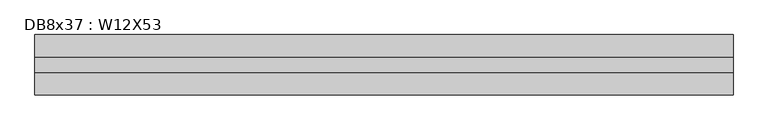
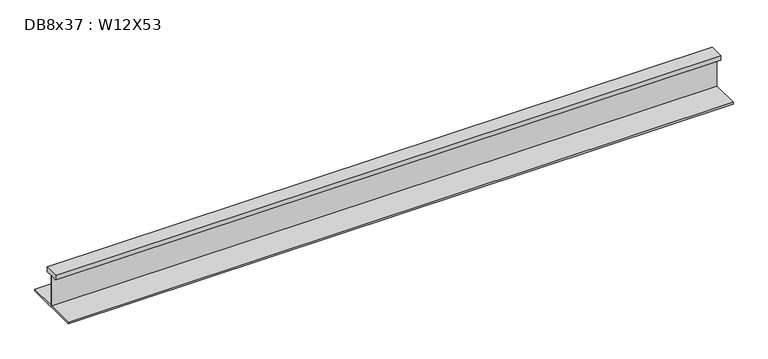
"""IFC4 building model written with IfcOpenShell, lengths in millimetres: beam geometry, DB8x37 : W12X53."""

import ifcopenshell
import ifcopenshell.guid

model = None  # the IFC model being written
_history = None  # IfcOwnerHistory: only IFC2X3 demands one
_inside = {}  # id of a spatial element -> (the spatial element, [elements in it])
_under = {}  # id of a project, library or spatial element -> (it, [spatial elements below it])
_declared = {}  # id of a project -> (the project, [libraries it declares])
_typed = {}  # id of a type object -> (the type object, [elements of that type])
_made_of = {}  # id of a material, layer set ... -> (it, [elements and type objects made of it])


def new_model(schema):
    """Start an empty IFC model of exactly this schema.

    Asked for "IFC4X3", IfcOpenShell would pick the latest addendum, in which some entities
    have other attributes; the version numbers below select the first issue.
    IFC2X3 requires an IfcOwnerHistory on every rooted entity: one is made here for all.
    """
    global model, _history
    if schema == "IFC4X3":
        model = ifcopenshell.file(schema_version=(4, 3, 0, 0))
    else:
        model = ifcopenshell.file(schema=schema)
    _inside.clear()
    _under.clear()
    _declared.clear()
    _typed.clear()
    _made_of.clear()
    _history = None
    if model.schema == "IFC2X3":
        org = make("IfcOrganization", Name="unknown")
        user = make(
            "IfcPersonAndOrganization",
            ThePerson=make("IfcPerson", FamilyName="unknown"),
            TheOrganization=org,
        )
        app = make(
            "IfcApplication",
            ApplicationDeveloper=org,
            Version="unknown",
            ApplicationFullName="unknown",
            ApplicationIdentifier="unknown",
        )
        _history = make(
            "IfcOwnerHistory",
            OwningUser=user,
            OwningApplication=app,
            ChangeAction="ADDED",
            CreationDate=0,
        )
    return model


def make(cls, **values):
    """One entity of the class cls with the attributes given. An attribute that is None is left unset."""
    return model.create_entity(
        cls, **{name: value for name, value in values.items() if value is not None}
    )


def rooted(cls, **values):
    """An entity with a GlobalId (a new one), such as an element, a storey or a relation."""
    return make(cls, GlobalId=ifcopenshell.guid.new(), OwnerHistory=_history, **values)


def si_unit(unit_type, name, prefix=None):
    """IfcSIUnit, for example si_unit("LENGTHUNIT", "METRE", prefix="MILLI")."""
    return make("IfcSIUnit", UnitType=unit_type, Prefix=prefix, Name=name)


def assignment(units):
    """IfcUnitAssignment: the units of a project."""
    return None if units is None else make("IfcUnitAssignment", Units=units)


def point(xyz):
    """IfcCartesianPoint."""
    return None if xyz is None else make("IfcCartesianPoint", Coordinates=xyz)


def direction(xyz):
    """IfcDirection."""
    return None if xyz is None else make("IfcDirection", DirectionRatios=xyz)


def frame(location, z_axis=None, x_axis=None):
    """IfcAxis2Placement3D, a coordinate frame: its origin and axes. An axis left out is left unset."""
    return make(
        "IfcAxis2Placement3D",
        Location=point(location),
        Axis=direction(z_axis),
        RefDirection=direction(x_axis),
    )


def origin():
    """The frame at (0, 0, 0) with its axes left unset."""
    return frame((0.0, 0.0, 0.0))


def place(relative_to, where):
    """IfcLocalPlacement: puts the frame where relative to a parent placement (None: the world)."""
    return make(
        "IfcLocalPlacement", PlacementRelTo=relative_to, RelativePlacement=where
    )


def context(
    kind, dimensions, precision=None, world=None, true_north=None, identifier=None
):
    """IfcGeometricRepresentationContext, for example the 3D "Model" context."""
    return make(
        "IfcGeometricRepresentationContext",
        ContextIdentifier=identifier,
        ContextType=kind,
        CoordinateSpaceDimension=dimensions,
        Precision=precision,
        WorldCoordinateSystem=world,
        TrueNorth=true_north,
    )


def project(units=None, contexts=None):
    """IfcProject with its units and contexts."""
    return rooted(
        "IfcProject",
        Name="project",
        RepresentationContexts=contexts,
        UnitsInContext=assignment(units),
    )


def spatial(cls, under=None, at=None, **own):
    """A site, building, storey or space (cls), placed at a placement, below another one or the project."""
    s = rooted(cls, ObjectPlacement=at, **own)
    if under is not None:
        _under.setdefault(under.id(), (under, []))[1].append(s)
    return s


def polyline(points):
    """IfcPolyline through the points."""
    return make("IfcPolyline", Points=[point(p) for p in points])


def outline(outer, holes=None, kind="AREA"):
    """IfcArbitraryClosedProfileDef: a profile drawn as a closed curve; with holes, ...WithVoids."""
    if holes is None:
        return make("IfcArbitraryClosedProfileDef", ProfileType=kind, OuterCurve=outer)
    return make(
        "IfcArbitraryProfileDefWithVoids",
        ProfileType=kind,
        OuterCurve=outer,
        InnerCurves=holes,
    )


def extrude(swept, where, along, depth):
    """IfcExtrudedAreaSolid: the profile swept, set in the frame where, extruded along a direction by depth."""
    return make(
        "IfcExtrudedAreaSolid",
        SweptArea=swept,
        Position=where,
        ExtrudedDirection=direction(along),
        Depth=depth,
    )


def shape(context_of_items, identifier, shape_type, items):
    """IfcShapeRepresentation: the items that make up one representation, for example the "Body"."""
    return make(
        "IfcShapeRepresentation",
        ContextOfItems=context_of_items,
        RepresentationIdentifier=identifier,
        RepresentationType=shape_type,
        Items=items,
    )


def source(mapping_origin, context_of_items, identifier, shape_type, items):
    """IfcRepresentationMap: a shape defined once, which mapped items show again and again."""
    return make(
        "IfcRepresentationMap",
        MappingOrigin=mapping_origin,
        MappedRepresentation=shape(context_of_items, identifier, shape_type, items),
    )


def transform(
    local_origin,
    x_axis=None,
    y_axis=None,
    z_axis=None,
    scale=None,
    scale2=None,
    scale3=None,
    uniform=True,
):
    """IfcCartesianTransformationOperator3D, or its non-uniform kind. x_axis, y_axis, z_axis: its Axis1, 2, 3."""
    if uniform:
        return make(
            "IfcCartesianTransformationOperator3D",
            Axis1=direction(x_axis),
            Axis2=direction(y_axis),
            LocalOrigin=point(local_origin),
            Scale=scale,
            Axis3=direction(z_axis),
        )
    return make(
        "IfcCartesianTransformationOperator3DnonUniform",
        Axis1=direction(x_axis),
        Axis2=direction(y_axis),
        LocalOrigin=point(local_origin),
        Scale=scale,
        Axis3=direction(z_axis),
        Scale2=scale2,
        Scale3=scale3,
    )


def mapped(mapping_source, mapping_target):
    """IfcMappedItem: shows the shape of a source again, moved by a transform."""
    return make(
        "IfcMappedItem", MappingSource=mapping_source, MappingTarget=mapping_target
    )


def made_of(thing, what):
    """Note that an element or type object is made of a material, layer set ...; save() writes the relation."""
    if what is not None:
        _made_of.setdefault(what.id(), (what, []))[1].append(thing)
    return thing


def element(
    cls,
    number,
    at=None,
    inside=None,
    cuts=None,
    type_object=None,
    material=None,
    context=None,
    identifier="Body",
    shape_type=None,
    held_by="IfcProductDefinitionShape",
    body=None,
    shapes=None,
    **own,
):
    """One element of the class cls, such as IfcWall. Its Tag is "e" and its number.

    at: its placement. inside: the storey or other place that contains it. cuts: it is an
    opening in that element (IfcRelVoidsElement). A single representation is given by context,
    identifier, shape_type and body (its items); several are given by shapes. held_by: the class
    of the entity that holds the representations. save() writes the other relations.
    """
    e = rooted(cls, Tag="e%d" % number, ObjectPlacement=at, **own)
    if body is not None:
        shapes = [shape(context, identifier, shape_type, body)]
    if shapes is not None:
        e.Representation = make(held_by, Representations=shapes)
    if inside is not None:
        _inside.setdefault(inside.id(), (inside, []))[1].append(e)
    if cuts is not None:
        rooted(
            "IfcRelVoidsElement", RelatingBuildingElement=cuts, RelatedOpeningElement=e
        )
    if type_object is not None:
        _typed.setdefault(type_object.id(), (type_object, []))[1].append(e)
    return made_of(e, material)


def aggregate(whole, parts):
    """IfcRelAggregates: a whole, such as a stair, and the parts it consists of."""
    return rooted("IfcRelAggregates", RelatingObject=whole, RelatedObjects=parts)


def save(model, path):
    """Write the relations noted so far, then the file.

    IfcRelAggregates (storeys below a building ...), IfcRelContainedInSpatialStructure (elements
    in a storey), IfcRelDefinesByType, IfcRelAssociatesMaterial and IfcRelDeclares: one each for
    every whole, place, type object, material and project.
    """
    for whole, parts in _under.values():
        aggregate(whole, parts)
    for where, things in _inside.values():
        rooted(
            "IfcRelContainedInSpatialStructure",
            RelatedElements=things,
            RelatingStructure=where,
        )
    for kind, things in _typed.values():
        rooted("IfcRelDefinesByType", RelatedObjects=things, RelatingType=kind)
    for what, things in _made_of.values():
        rooted("IfcRelAssociatesMaterial", RelatedObjects=things, RelatingMaterial=what)
    for by, libraries in _declared.values():
        rooted("IfcRelDeclares", RelatingContext=by, RelatedDefinitions=libraries)
    model.write(path)


def db8x37_w12x53_4f632cbe(model_context):
    return source(origin(), model_context, "Body", "SweptSolid", [
        extrude(outline(polyline([(38.1, 145.415), (38.1, 120.015), (2.921, 120.015), (2.921, -48.4505), (152.4, -48.4505), (152.4, -58.1025), (-152.4, -58.1025), (-152.4, -48.4505), (-2.921, -48.4505), (-2.921, 120.015), (-38.1, 120.015), (-38.1, 145.415), (38.1, 145.415)])), frame((-1760.9030956, 0.0, 0.0), z_axis=(1.0, 0.0, 0.0), x_axis=(0.0, 1.0, 0.0)), (0.0, 0.0, 1.0), 3528.892742),
    ])


if __name__ == "__main__":
    model = new_model("IFC4")
    model_context = context("Model", 3, world=origin())
    ifc_project = project(units=[si_unit("LENGTHUNIT", "METRE", prefix="MILLI")], contexts=[model_context])
    site = spatial("IfcSite", under=ifc_project)
    building = spatial("IfcBuilding", under=site)
    placement = place(None, origin())
    db8x37_w12x53_shape = db8x37_w12x53_4f632cbe(model_context)
    element("IfcBeam", 1, ObjectType="DB8x37 : W12X53", at=placement, inside=building, context=model_context, shape_type="MappedRepresentation", body=[
        mapped(db8x37_w12x53_shape, transform((0.0, 0.0, 0.0), x_axis=(1.0, 0.0, 0.0), y_axis=(0.0, 1.0, 0.0), z_axis=(0.0, 0.0, 1.0))),
    ])
    save(model, "model.ifc")

# Revit data of these elements
# Type "DB8x37 : W12X53"
#   Assembly Code = "B10"
#   W = 53
#   Length [instance default] = 5' - 0"
#   bf = 0' - 10"
#   d = 1' - 0.1"
#   k = 0' - 1 3/8"
#   k2 = 0' - 0.8"
#   tf = 0' - 0.575"
#   tw = 0' - 0.345"
#   A = 0.108333 SF
#   Structural Material [instance default] = Steel ASTM A992
# Element 1 (IfcBeam, "DB8x37 : W12X53")
#   Materials on its faces: "Steel ASTM A992"
# Materials
#   "Steel ASTM A992": class "Metal", colour RGB 199 199 199, transparency 0, Description = "Structural steel 50ksi", Cost = 0
